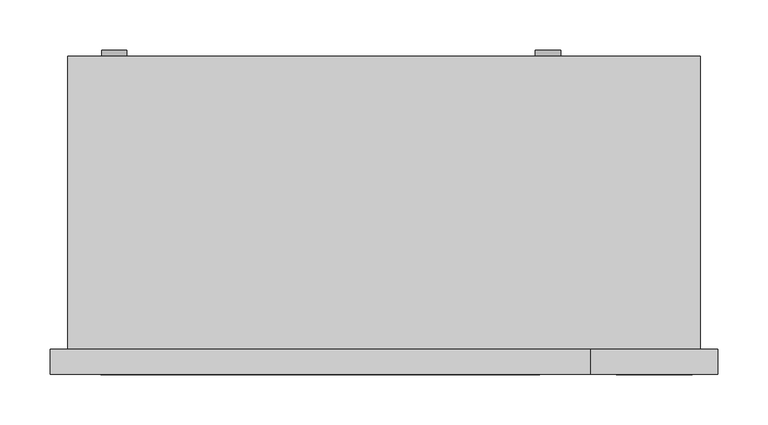
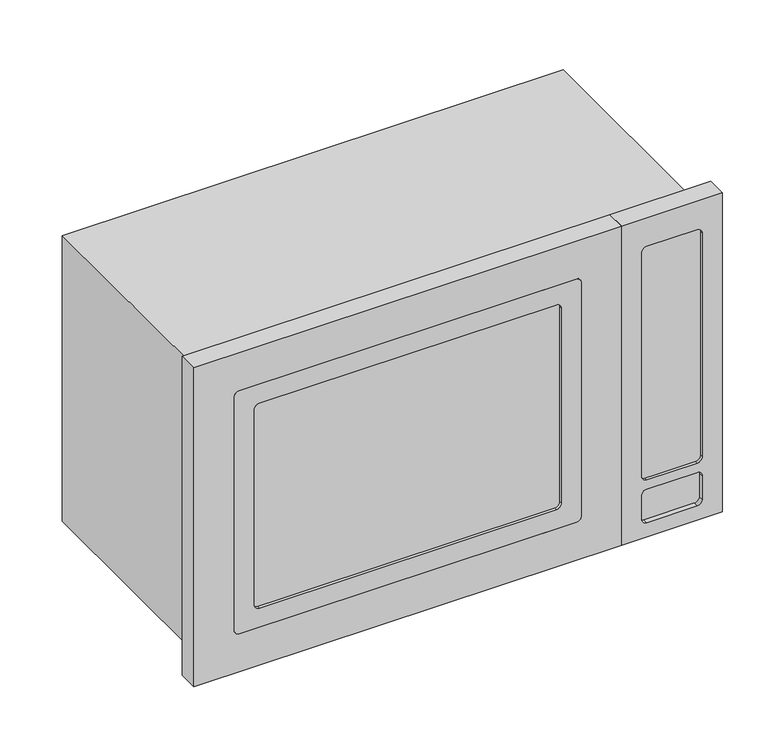
"""IFC4 building model written with IfcOpenShell, lengths in millimetres: proxy geometry, Microwave_Compact-Ovens_GE-Monogram_ZEM200SF : Microwave_Compact-Ovens_GE-Monogram_ZEM200SF."""

from ifc_helpers import new_model, si_unit, point, frame, frame_2d, origin, place, context, project, spatial, polyline, circle_curve, trimmed, segment, composite_curve, outline, extrude, source, transform, mapped, element, save
from ifc_brep_helpers import plane_surface, revolved_surface, advanced_brep


def specialty_equipment_f386db1e(model_context):
    return source(origin(), model_context, "Body", "SolidModel", [
        extrude(outline(composite_curve([segment(trimmed(circle_curve(frame_2d((368.3, -276.225)), 6.35), [point((374.65, -276.225))], [point((368.3, -282.575))], False, "CARTESIAN"), True, "CONTINUOUS"), segment(polyline([(368.3, -282.575), (57.15, -282.575)]), True, "CONTINUOUS"), segment(trimmed(circle_curve(frame_2d((57.15, -276.225)), 6.35), [point((57.15, -282.575))], [point((50.8, -276.225))], False, "CARTESIAN"), True, "CONTINUOUS"), segment(polyline([(50.8, -276.225), (50.8, 149.225)]), True, "CONTINUOUS"), segment(trimmed(circle_curve(frame_2d((57.15, 149.225)), 6.35), [point((50.8, 149.225))], [point((57.15, 155.575))], False, "CARTESIAN"), True, "CONTINUOUS"), segment(polyline([(57.15, 155.575), (368.3, 155.575)]), True, "CONTINUOUS"), segment(trimmed(circle_curve(frame_2d((368.3, 149.225)), 6.35), [point((368.3, 155.575))], [point((374.65, 149.225))], False, "CARTESIAN"), True, "CONTINUOUS"), segment(polyline([(374.65, 149.225), (374.65, -276.225)]), True, "CONTINUOUS")], self_intersect=False), holes=[composite_curve([segment(trimmed(circle_curve(frame_2d((342.9, -250.825)), 6.35), [point((342.9, -257.175))], [point((349.25, -250.825))], True, "CARTESIAN"), True, "CONTINUOUS"), segment(polyline([(349.25, -250.825), (349.25, 123.825)]), True, "CONTINUOUS"), segment(trimmed(circle_curve(frame_2d((342.9, 123.825)), 6.35), [point((349.25, 123.825))], [point((342.9, 130.175))], True, "CARTESIAN"), True, "CONTINUOUS"), segment(polyline([(342.9, 130.175), (82.55, 130.175)]), True, "CONTINUOUS"), segment(trimmed(circle_curve(frame_2d((82.55, 123.825)), 6.35), [point((82.55, 130.175))], [point((76.2, 123.825))], True, "CARTESIAN"), True, "CONTINUOUS"), segment(polyline([(76.2, 123.825), (76.2, -250.825)]), True, "CONTINUOUS"), segment(trimmed(circle_curve(frame_2d((82.55, -250.825)), 6.35), [point((76.2, -250.825))], [point((82.55, -257.175))], True, "CARTESIAN"), True, "CONTINUOUS"), segment(polyline([(82.55, -257.175), (342.9, -257.175)]), True, "CONTINUOUS")], self_intersect=False)]), frame((0.0, -69.85, 0.0), z_axis=(0.0, 1.0, 0.0), x_axis=(0.0, 0.0, 1.0)), (0.0, 0.0, 1.0), 6.35),
        advanced_brep(
        [(333.375, -44.45, 425.45), (333.375, -44.45, 0.0), (206.375, -44.45, 0.0), (206.375, -44.45, 425.45), (333.375, -69.85, 425.45), (206.375, -69.85, 425.45), (206.375, -69.85, 0.0), (333.375, -69.85, 0.0), (307.975, -69.85, 82.55), (301.625, -69.85, 76.2), (238.125, -69.85, 76.2), (231.775, -69.85, 82.55), (231.775, -69.85, 381.0), (238.125, -69.85, 387.35), (301.625, -69.85, 387.35), (307.975, -69.85, 381.0), (301.625, -69.85, 63.5), (307.975, -69.85, 57.15), (307.975, -69.85, 25.4), (301.625, -69.85, 19.05), (238.125, -69.85, 19.05), (231.775, -69.85, 25.4), (231.775, -69.85, 57.15), (238.125, -69.85, 63.5), (307.975, -63.5, 82.55), (307.975, -63.5, 381.0), (301.625, -63.5, 387.35), (238.125, -63.5, 387.35), (231.775, -63.5, 381.0), (231.775, -63.5, 82.55), (238.125, -63.5, 76.2), (301.625, -63.5, 76.2), (301.625, -63.5, 63.5), (238.125, -63.5, 63.5), (231.775, -63.5, 57.15), (231.775, -63.5, 25.4), (238.125, -63.5, 19.05), (301.625, -63.5, 19.05), (307.975, -63.5, 25.4), (307.975, -63.5, 57.15)],
        [
            (0, 1),
            (1, 2),
            (2, 3),
            (3, 0),
            (4, 5),
            (5, 6),
            (6, 7),
            (7, 4),
            (8, 9, circle_curve(frame((301.625, -69.85, 82.55), z_axis=(0.0, 1.0, 0.0), x_axis=(-1.0, 0.0, 0.0)), 6.35)),
            (9, 10),
            (10, 11, circle_curve(frame((238.125, -69.85, 82.55), z_axis=(0.0, 1.0, 0.0), x_axis=(-1.0, 0.0, 0.0)), 6.35)),
            (11, 12),
            (12, 13, circle_curve(frame((238.125, -69.85, 381.0), z_axis=(0.0, 1.0, 0.0), x_axis=(-1.0, 0.0, 0.0)), 6.35)),
            (13, 14),
            (14, 15, circle_curve(frame((301.625, -69.85, 381.0), z_axis=(0.0, 1.0, 0.0), x_axis=(-1.0, 0.0, 0.0)), 6.35)),
            (15, 8),
            (16, 17, circle_curve(frame((301.625, -69.85, 57.15), z_axis=(0.0, 1.0, 0.0), x_axis=(-1.0, 0.0, 0.0)), 6.35)),
            (17, 18),
            (18, 19, circle_curve(frame((301.625, -69.85, 25.4), z_axis=(0.0, 1.0, 0.0), x_axis=(-1.0, 0.0, 0.0)), 6.35)),
            (19, 20),
            (20, 21, circle_curve(frame((238.125, -69.85, 25.4), z_axis=(0.0, 1.0, 0.0), x_axis=(-1.0, 0.0, 0.0)), 6.35)),
            (21, 22),
            (22, 23, circle_curve(frame((238.125, -69.85, 57.15), z_axis=(0.0, 1.0, 0.0), x_axis=(-1.0, 0.0, 0.0)), 6.35)),
            (23, 16),
            (0, 4),
            (7, 1),
            (6, 2),
            (5, 3),
            (24, 25),
            (25, 26, circle_curve(frame((301.625, -63.5, 381.0), z_axis=(0.0, -1.0, 0.0), x_axis=(-1.0, 0.0, 0.0)), 6.35)),
            (26, 27),
            (27, 28, circle_curve(frame((238.125, -63.5, 381.0), z_axis=(0.0, -1.0, 0.0), x_axis=(-1.0, 0.0, 0.0)), 6.35)),
            (28, 29),
            (29, 30, circle_curve(frame((238.125, -63.5, 82.55), z_axis=(0.0, -1.0, 0.0), x_axis=(-1.0, 0.0, 0.0)), 6.35)),
            (30, 31),
            (31, 24, circle_curve(frame((301.625, -63.5, 82.55), z_axis=(0.0, -1.0, 0.0), x_axis=(-1.0, 0.0, 0.0)), 6.35)),
            (32, 33),
            (33, 34, circle_curve(frame((238.125, -63.5, 57.15), z_axis=(0.0, -1.0, 0.0), x_axis=(-1.0, 0.0, 0.0)), 6.35)),
            (34, 35),
            (35, 36, circle_curve(frame((238.125, -63.5, 25.4), z_axis=(0.0, -1.0, 0.0), x_axis=(-1.0, 0.0, 0.0)), 6.35)),
            (36, 37),
            (37, 38, circle_curve(frame((301.625, -63.5, 25.4), z_axis=(0.0, -1.0, 0.0), x_axis=(-1.0, 0.0, 0.0)), 6.35)),
            (38, 39),
            (39, 32, circle_curve(frame((301.625, -63.5, 57.15), z_axis=(0.0, -1.0, 0.0), x_axis=(-1.0, 0.0, 0.0)), 6.35)),
            (31, 9),
            (8, 24),
            (30, 10),
            (29, 11),
            (28, 12),
            (27, 13),
            (26, 14),
            (25, 15),
            (39, 17),
            (16, 32),
            (38, 18),
            (37, 19),
            (36, 20),
            (35, 21),
            (34, 22),
            (33, 23),
        ],
        [
            plane_surface(frame((333.375, -44.45, 425.45), z_axis=(0.0, 1.0, 0.0), x_axis=(0.0, 0.0, -1.0))),
            plane_surface(frame((333.375, -69.85, 425.45), z_axis=(0.0, -1.0, 0.0), x_axis=(0.0, 0.0, 1.0))),
            plane_surface(frame((333.375, -44.45, 425.45), z_axis=(1.0, 0.0, 0.0), x_axis=(0.0, -1.0, 0.0))),
            plane_surface(frame((333.375, -44.45, 0.0), z_axis=(0.0, 0.0, -1.0), x_axis=(0.0, -1.0, 0.0))),
            plane_surface(frame((206.375, -44.45, 0.0), z_axis=(-1.0, 0.0, 0.0), x_axis=(0.0, -1.0, 0.0))),
            plane_surface(frame((206.375, -44.45, 425.45), z_axis=(0.0, 0.0, 1.0), x_axis=(0.0, -1.0, 0.0))),
            plane_surface(frame((295.275, -63.5, 82.55), z_axis=(0.0, -1.0, 0.0), x_axis=(0.0, 0.0, 1.0))),
            revolved_surface(polyline([(295.275, -63.5, 82.55), (295.275, -69.85, 82.55)]), (301.625, -69.85, 82.55), (0.0, 1.0, 0.0)),
            plane_surface(frame((301.625, -63.5, 76.2), z_axis=(0.0, 0.0, 1.0), x_axis=(0.0, -1.0, 0.0))),
            revolved_surface(polyline([(231.775, -63.5, 82.55), (231.775, -69.85, 82.55)]), (238.125, -69.85, 82.55), (0.0, 1.0, 0.0)),
            plane_surface(frame((231.775, -63.5, 82.55), z_axis=(1.0, 0.0, 0.0), x_axis=(0.0, -1.0, 0.0))),
            revolved_surface(polyline([(231.775, -63.5, 381.0), (231.775, -69.85, 381.0)]), (238.125, -69.85, 381.0), (0.0, 1.0, 0.0)),
            plane_surface(frame((238.125, -63.5, 387.35), z_axis=(0.0, 0.0, -1.0), x_axis=(0.0, -1.0, 0.0))),
            revolved_surface(polyline([(295.275, -63.5, 381.0), (295.275, -69.85, 381.0)]), (301.625, -69.85, 381.0), (0.0, 1.0, 0.0)),
            plane_surface(frame((307.975, -63.5, 381.0), z_axis=(-1.0, 0.0, 0.0), x_axis=(0.0, -1.0, 0.0))),
            revolved_surface(polyline([(295.275, -63.5, 57.15), (295.275, -69.85, 57.15)]), (301.625, -69.85, 57.15), (0.0, 1.0, 0.0)),
            plane_surface(frame((307.975, -63.5, 57.15), z_axis=(-1.0, 0.0, 0.0), x_axis=(0.0, -1.0, 0.0))),
            revolved_surface(polyline([(295.275, -63.5, 25.4), (295.275, -69.85, 25.4)]), (301.625, -69.85, 25.4), (0.0, 1.0, 0.0)),
            plane_surface(frame((301.625, -63.5, 19.05), z_axis=(0.0, 0.0, 1.0), x_axis=(0.0, -1.0, 0.0))),
            revolved_surface(polyline([(231.775, -63.5, 25.4), (231.775, -69.85, 25.4)]), (238.125, -69.85, 25.4), (0.0, 1.0, 0.0)),
            plane_surface(frame((231.775, -63.5, 25.4), z_axis=(1.0, 0.0, 0.0), x_axis=(0.0, -1.0, 0.0))),
            revolved_surface(polyline([(231.775, -63.5, 57.15), (231.775, -69.85, 57.15)]), (238.125, -69.85, 57.15), (0.0, 1.0, 0.0)),
            plane_surface(frame((238.125, -63.5, 63.5), z_axis=(0.0, 0.0, -1.0), x_axis=(0.0, -1.0, 0.0))),
        ],
        [
            (0, [[1, 2, 3, 4]]),
            (1, [[5, 6, 7, 8], [9, 10, 11, 12, 13, 14, 15, 16], [17, 18, 19, 20, 21, 22, 23, 24]]),
            (2, [[-1, 25, -8, 26]]),
            (3, [[-2, -26, -7, 27]]),
            (4, [[-3, -27, -6, 28]]),
            (5, [[-4, -28, -5, -25]]),
            (6, [[29, 30, 31, 32, 33, 34, 35, 36]]),
            (6, [[37, 38, 39, 40, 41, 42, 43, 44]]),
            (7, [[-36, 45, -9, 46]]),
            (8, [[-35, 47, -10, -45]]),
            (9, [[-34, 48, -11, -47]]),
            (10, [[-33, 49, -12, -48]]),
            (11, [[-32, 50, -13, -49]]),
            (12, [[-31, 51, -14, -50]]),
            (13, [[-30, 52, -15, -51]]),
            (14, [[-29, -46, -16, -52]]),
            (15, [[-44, 53, -17, 54]]),
            (16, [[-43, 55, -18, -53]]),
            (17, [[-42, 56, -19, -55]]),
            (18, [[-41, 57, -20, -56]]),
            (19, [[-40, 58, -21, -57]]),
            (20, [[-39, 59, -22, -58]]),
            (21, [[-38, 60, -23, -59]]),
            (22, [[-37, -54, -24, -60]]),
        ],
    ),
        advanced_brep(
        [(206.375, -44.45, 425.45), (206.375, -44.45, 0.0), (-333.375, -44.45, 0.0), (-333.375, -44.45, 425.45), (206.375, -69.85, 425.45), (-333.375, -69.85, 425.45), (-333.375, -69.85, 0.0), (206.375, -69.85, 0.0), (-282.575, -69.85, 57.15), (-282.575, -69.85, 368.3), (-276.225, -69.85, 374.65), (149.225, -69.85, 374.65), (155.575, -69.85, 368.3), (155.575, -69.85, 57.15), (149.225, -69.85, 50.8), (-276.225, -69.85, 50.8), (-276.225, -63.5, 50.8), (149.225, -63.5, 50.8), (155.575, -63.5, 57.15), (155.575, -63.5, 368.3), (149.225, -63.5, 374.65), (-276.225, -63.5, 374.65), (-282.575, -63.5, 368.3), (-282.575, -63.5, 57.15)],
        [
            (0, 1),
            (1, 2),
            (2, 3),
            (3, 0),
            (4, 5),
            (5, 6),
            (6, 7),
            (7, 4),
            (8, 9),
            (9, 10, circle_curve(frame((-276.225, -69.85, 368.3), z_axis=(0.0, 1.0, 0.0), x_axis=(-1.0, 0.0, 0.0)), 6.35)),
            (10, 11),
            (11, 12, circle_curve(frame((149.225, -69.85, 368.3), z_axis=(0.0, 1.0, 0.0), x_axis=(-1.0, 0.0, 0.0)), 6.35)),
            (12, 13),
            (13, 14, circle_curve(frame((149.225, -69.85, 57.15), z_axis=(0.0, 1.0, 0.0), x_axis=(-1.0, 0.0, 0.0)), 6.35)),
            (14, 15),
            (15, 8, circle_curve(frame((-276.225, -69.85, 57.15), z_axis=(0.0, 1.0, 0.0), x_axis=(-1.0, 0.0, 0.0)), 6.35)),
            (0, 4),
            (7, 1),
            (6, 2),
            (5, 3),
            (16, 17),
            (17, 18, circle_curve(frame((149.225, -63.5, 57.15), z_axis=(0.0, -1.0, 0.0), x_axis=(-1.0, 0.0, 0.0)), 6.35)),
            (18, 19),
            (19, 20, circle_curve(frame((149.225, -63.5, 368.3), z_axis=(0.0, -1.0, 0.0), x_axis=(-1.0, 0.0, 0.0)), 6.35)),
            (20, 21),
            (21, 22, circle_curve(frame((-276.225, -63.5, 368.3), z_axis=(0.0, -1.0, 0.0), x_axis=(-1.0, 0.0, 0.0)), 6.35)),
            (22, 23),
            (23, 16, circle_curve(frame((-276.225, -63.5, 57.15), z_axis=(0.0, -1.0, 0.0), x_axis=(-1.0, 0.0, 0.0)), 6.35)),
            (23, 8),
            (15, 16),
            (22, 9),
            (21, 10),
            (20, 11),
            (19, 12),
            (18, 13),
            (17, 14),
        ],
        [
            plane_surface(frame((206.375, -44.45, 425.45), z_axis=(0.0, 1.0, 0.0), x_axis=(0.0, 0.0, -1.0))),
            plane_surface(frame((206.375, -69.85, 425.45), z_axis=(0.0, -1.0, 0.0), x_axis=(0.0, 0.0, 1.0))),
            plane_surface(frame((206.375, -44.45, 425.45), z_axis=(1.0, 0.0, 0.0), x_axis=(0.0, -1.0, 0.0))),
            plane_surface(frame((206.375, -44.45, 0.0), z_axis=(0.0, 0.0, -1.0), x_axis=(0.0, -1.0, 0.0))),
            plane_surface(frame((-333.375, -44.45, 0.0), z_axis=(-1.0, 0.0, 0.0), x_axis=(0.0, -1.0, 0.0))),
            plane_surface(frame((-333.375, -44.45, 425.45), z_axis=(0.0, 0.0, 1.0), x_axis=(0.0, -1.0, 0.0))),
            plane_surface(frame((-282.575, -63.5, 57.15), z_axis=(0.0, -1.0, 0.0), x_axis=(0.0, 0.0, 1.0))),
            revolved_surface(polyline([(-282.57500000000005, -63.5, 57.15), (-282.57500000000005, -69.85, 57.15)]), (-276.225, -69.85, 57.15), (0.0, 1.0, 0.0)),
            plane_surface(frame((-282.575, -63.5, 57.15), z_axis=(1.0, 0.0, 0.0), x_axis=(0.0, -1.0, 0.0))),
            revolved_surface(polyline([(-282.57500000000005, -63.5, 368.3), (-282.57500000000005, -69.85, 368.3)]), (-276.225, -69.85, 368.3), (0.0, 1.0, 0.0)),
            plane_surface(frame((-276.225, -63.5, 374.65), z_axis=(0.0, 0.0, -1.0), x_axis=(0.0, -1.0, 0.0))),
            revolved_surface(polyline([(142.875, -63.5, 368.3), (142.875, -69.85, 368.3)]), (149.225, -69.85, 368.3), (0.0, 1.0, 0.0)),
            plane_surface(frame((155.575, -63.5, 368.3), z_axis=(-1.0, 0.0, 0.0), x_axis=(0.0, -1.0, 0.0))),
            revolved_surface(polyline([(142.875, -63.5, 57.15), (142.875, -69.85, 57.15)]), (149.225, -69.85, 57.15), (0.0, 1.0, 0.0)),
            plane_surface(frame((149.225, -63.5, 50.8), z_axis=(0.0, 0.0, 1.0), x_axis=(0.0, -1.0, 0.0))),
        ],
        [
            (0, [[1, 2, 3, 4]]),
            (1, [[5, 6, 7, 8], [9, 10, 11, 12, 13, 14, 15, 16]]),
            (2, [[-1, 17, -8, 18]]),
            (3, [[-2, -18, -7, 19]]),
            (4, [[-3, -19, -6, 20]]),
            (5, [[-4, -20, -5, -17]]),
            (6, [[21, 22, 23, 24, 25, 26, 27, 28]]),
            (7, [[-28, 29, -16, 30]]),
            (8, [[-27, 31, -9, -29]]),
            (9, [[-26, 32, -10, -31]]),
            (10, [[-25, 33, -11, -32]]),
            (11, [[-24, 34, -12, -33]]),
            (12, [[-23, 35, -13, -34]]),
            (13, [[-22, 36, -14, -35]]),
            (14, [[-21, -30, -15, -36]]),
        ],
    ),
        extrude(outline(composite_curve([segment(polyline([(349.25, 123.825), (349.25, -250.825)]), True, "CONTINUOUS"), segment(trimmed(circle_curve(frame_2d((342.9, -250.825)), 6.35), [point((349.25, -250.825))], [point((342.9, -257.175))], False, "CARTESIAN"), True, "CONTINUOUS"), segment(polyline([(342.9, -257.175), (82.55, -257.175)]), True, "CONTINUOUS"), segment(trimmed(circle_curve(frame_2d((82.55, -250.825)), 6.35), [point((82.55, -257.175))], [point((76.2, -250.825))], False, "CARTESIAN"), True, "CONTINUOUS"), segment(polyline([(76.2, -250.825), (76.2, 123.825)]), True, "CONTINUOUS"), segment(trimmed(circle_curve(frame_2d((82.55, 123.825)), 6.35), [point((76.2, 123.825))], [point((82.55, 130.175))], False, "CARTESIAN"), True, "CONTINUOUS"), segment(polyline([(82.55, 130.175), (342.9, 130.175)]), True, "CONTINUOUS"), segment(trimmed(circle_curve(frame_2d((342.9, 123.825)), 6.35), [point((342.9, 130.175))], [point((349.25, 123.825))], False, "CARTESIAN"), True, "CONTINUOUS")], self_intersect=False)), frame((0.0, -66.675, 0.0), z_axis=(0.0, 1.0, 0.0), x_axis=(0.0, 0.0, 1.0)), (0.0, 0.0, 1.0), 3.175),
        extrude(outline(composite_curve([segment(trimmed(circle_curve(frame_2d((381.0, 238.125)), 6.35), [point((387.35, 238.125))], [point((381.0, 231.775))], False, "CARTESIAN"), True, "CONTINUOUS"), segment(polyline([(381.0, 231.775), (82.55, 231.775)]), True, "CONTINUOUS"), segment(trimmed(circle_curve(frame_2d((82.55, 238.125)), 6.35), [point((82.55, 231.775))], [point((76.2, 238.125))], False, "CARTESIAN"), True, "CONTINUOUS"), segment(polyline([(76.2, 238.125), (76.2, 301.625)]), True, "CONTINUOUS"), segment(trimmed(circle_curve(frame_2d((82.55, 301.625)), 6.35), [point((76.2, 301.625))], [point((82.55, 307.975))], False, "CARTESIAN"), True, "CONTINUOUS"), segment(polyline([(82.55, 307.975), (381.0, 307.975)]), True, "CONTINUOUS"), segment(trimmed(circle_curve(frame_2d((381.0, 301.625)), 6.35), [point((381.0, 307.975))], [point((387.35, 301.625))], False, "CARTESIAN"), True, "CONTINUOUS"), segment(polyline([(387.35, 301.625), (387.35, 238.125)]), True, "CONTINUOUS")], self_intersect=False)), frame((0.0, -66.675, 0.0), z_axis=(0.0, 1.0, 0.0), x_axis=(0.0, 0.0, 1.0)), (0.0, 0.0, 1.0), 3.175),
        extrude(outline(polyline([(315.9125, -44.45), (-315.9125, -44.45), (-315.9125, 247.65), (315.9125, 247.65), (315.9125, -44.45)])), frame((0.0, 0.0, 22.225), z_axis=(0.0, 0.0, 1.0), x_axis=(1.0, 0.0, 0.0)), (0.0, 0.0, 1.0), 381.0),
        extrude(outline(composite_curve([segment(trimmed(circle_curve(frame_2d((314.6288473, -269.2820411)), 12.7), [point((314.6288473, -256.5820411))], [point((314.6288473, -281.9820411))], False, "CARTESIAN"), True, "CONTINUOUS"), segment(trimmed(circle_curve(frame_2d((314.6288473, -269.2820411)), 12.7), [point((314.6288473, -281.9820411))], [point((314.6288473, -256.5820411))], False, "CARTESIAN"), True, "CONTINUOUS")], self_intersect=False)), frame((0.0, 247.65, 0.0), z_axis=(0.0, 1.0, 0.0), x_axis=(0.0, 0.0, 1.0)), (0.0, 0.0, 1.0), 6.35),
        extrude(outline(composite_curve([segment(trimmed(circle_curve(frame_2d((314.6288473, 163.6862686)), 12.7), [point((314.6288473, 176.3862686))], [point((314.6288473, 150.9862686))], False, "CARTESIAN"), True, "CONTINUOUS"), segment(trimmed(circle_curve(frame_2d((314.6288473, 163.6862686)), 12.7), [point((314.6288473, 150.9862686))], [point((314.6288473, 176.3862686))], False, "CARTESIAN"), True, "CONTINUOUS")], self_intersect=False)), frame((0.0, 247.65, 0.0), z_axis=(0.0, 1.0, 0.0), x_axis=(0.0, 0.0, 1.0)), (0.0, 0.0, 1.0), 6.35),
    ])


if __name__ == "__main__":
    model = new_model("IFC4")
    model_context = context("Model", 3, world=origin())
    ifc_project = project(units=[si_unit("LENGTHUNIT", "METRE", prefix="MILLI")], contexts=[model_context])
    site = spatial("IfcSite", under=ifc_project)
    building = spatial("IfcBuilding", under=site)
    placement = place(None, origin())
    specialty_equipment_shape = specialty_equipment_f386db1e(model_context)
    element("IfcBuildingElementProxy", 1, Name="Microwave_Compact-Ovens_GE-Monogram_ZEM200SF : Microwave_Compact-Ovens_GE-Monogram_ZEM200SF", ObjectType="Microwave_Compact-Ovens_GE-Monogram_ZEM200SF : Microwave_Compact-Ovens_GE-Monogram_ZEM200SF", at=placement, inside=building, context=model_context, shape_type="MappedRepresentation", body=[
        mapped(specialty_equipment_shape, transform((0.0, 0.0, 0.0), x_axis=(1.0, 0.0, 0.0), y_axis=(0.0, 1.0, 0.0), z_axis=(0.0, 0.0, 1.0))),
    ])
    save(model, "model.ifc")

# Revit data of these elements
# Type "Microwave_Compact-Ovens_GE-Monogram_ZEM200SF : Microwave_Compact-Ovens_GE-Monogram_ZEM200SF"
#   COBie.Type.CreatedBy = "design@eagle.com"
#   COBie.Type.CreatedOn = "2016-10-27T05:31:12"
#   COBie.Type.Name = "Microwave_Compact-Ovens_GE-Monogram_ZEM200SF_Microwave_Compact-Ovens_GE-Monogram_ZEM200SF"
#   COBie.Type.Category = "23-40 40 14 17 11 : Cookers, Ovens, Stoves"
#   COBie.Type.Description = "Microwave_Compact-Ovens_GE-Monogram_ZEM200SF_Microwave_Compact-Ovens_GE-Monogram_ZEM200SF"
#   COBie.Type.Manufacturer = "info@geappliances.com"
#   COBie.Type.ModelNumber = "As Specified in 11 30 00"
#   URL = "http://www.geappliances.com/"
#   Test Data = "http://www.geappliances.com/service_and_support/search.htm"
#   Specification = "http://www.arcat.com/sdspecs/htm/11450gea.htm"
#   SpecWizard = "http://www.arcat.com/specwizard/11450gea/index.htm?mf=&coid=32703"
#   Send Message = "http://www.arcat.com/users.pl?action=UserEmail&company=GE%20Appliances&coid=32703&rep=114&fax=502-452-0620&mf="
#   Sales Information = "http://www.geappliances.com/buy/"
#   Revision = "R1_02-2011"
#   Product Properties = "http://www.arcat.com/bim/bim_info.pl?fn=GEAppliances"
#   Product Data = "http://www.arcat.com/arcatcos/cos32/arc32703.html"
#   Model = "As Specified in 11 30 00"
#   Manufacturer Website = "http://www.geappliances.com/"
#   Manufacturer Phone - Toll Free = "800-626-2000"
#   Manufacturer Phone = "502-452-3346"
#   Manufacturer Fax = "502-452-0620"
#   Manufacturer Address = "Appliance Park AP4-109, Louisville, KY 40225"
#   Manufacturer = "info@geappliances.com"
#   Keynote = "11 30 00"
#   Installation-Fabrication = "http://www.geappliances.com/service_and_support/literature/"
#   Installation Phase = ""
#   Heat Source = ""
#   Green Building-LEED = "http://www.geappliances.com/energy-star-appliances/"
#   ENERGYSTAR Qualified = ""
#   Drawn By = "Sumex Design, Inc. / Robert S. Weygant, CSI, CDT, SCIP"
#   Description = "Residential Appliance as Specified in 11 30 00"
#   Copyright = "©Arcat Inc."
#   Cooktop Type = ""
#   Cooking Technology = ""
#   Construction Details = "http://www.geappliances.com/design_center/"
#   Building Codes = "http://www.geappliances.com/service_and_support/search.htm"
#   Assembly Code = "E1090400"
#   COBie.Type.ReplacementCost = 0
#   offset [instance default] = 0' - 0"
#   Voltage_MEP = 120 V
#   Unit Width = 2' - 2 1/4"
#   Unit Height = 1' - 4 3/4"
#   Unit Depth = 1' - 0 1/2"
#   MEP Apparent Power = 60 VA
#   MEP Amperage = 0.5 A
#   HWRad = 0' - 0 1/4"
#   GasRad = 0' - 0 1/4"
#   DrainRad = 0' - 0 5/8"
#   Connection Dia HW = 0' - 0 1/2"
#   Connection Dia Gas = 0' - 0 1/2"
#   Connection Dia DWV = 0' - 1 1/4"
#   Connection Dia CW = 0' - 0 1/2"
#   CWRad = 0' - 0 1/4"
#   COBie.Type = yes
#   Warranty Duration (Years) = 0
#   Self Cleaning = yes
#   Maintenance Schedule (Months) = 0
#   Expected Lifespan (Years) = 0
#   ADA Compliant = yes
#   Glass = Glass
#   Exterior Finish = ARCAT - Metal - Aluminum_0.032" - White
# Element 1 (IfcBuildingElementProxy, "Microwave_Compact-Ovens_GE-Monogram_ZEM200SF : Microwave_Compact-Ovens_GE-Monogram_ZEM200SF")
#   Materials on its faces: "ARCAT - Metal - Aluminum_0.032\" - White", "Glass", "Gas", "Connector"
# Materials
#   "Glass": class "Glass", colour RGB 0 128 192, transparency 0.75, Description = "Soda Lime Glass", Cost = 0
#   "ARCAT - Metal - Aluminum_0.032\" - White": class "Unassigned", colour RGB 249 249 249, transparency 0, Keynote = "05050", Model = "Generic", Manufacturer = "Generic", Description = "Aluminum, 0.032\""
#   "Gas": class "Miscellaneous", colour RGB 255 0 255, transparency 0
#   "Connector": class "Miscellaneous", colour RGB 255 255 0, transparency 0
